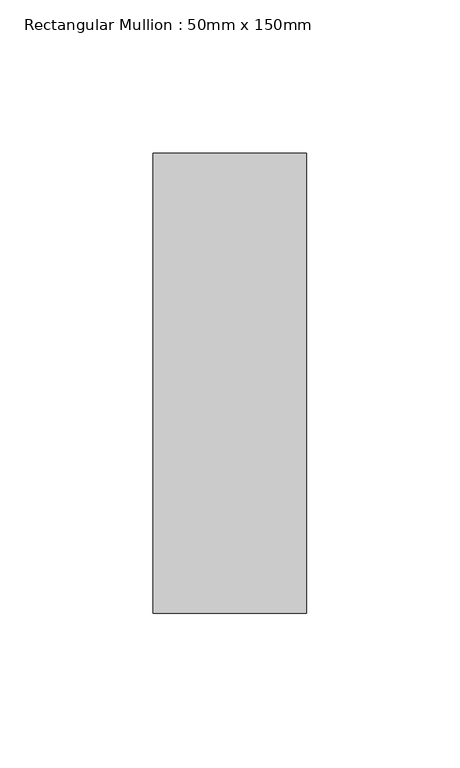
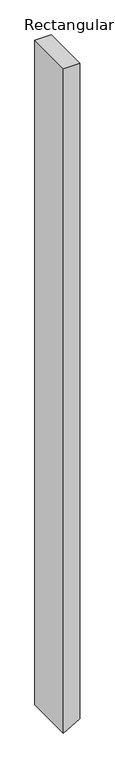
"""IFC4 building model written with IfcOpenShell, lengths in millimetres: member geometry, Rectangular Mullion : 50mm x 150mm."""

from ifc_helpers import new_model, si_unit, frame, origin, place, context, project, spatial, polyline, outline, extrude, source, transform, mapped, element, save


def rectangular_mullion_50mm_x_150mm_c4d7f9a4(model_context):
    return source(origin(), model_context, "Body", "SweptSolid", [
        extrude(outline(polyline([(0.0, 25.0), (0.0, -25.0), (-2134.1765467, -25.0), (-2105.3090332, 25.0), (0.0, 25.0)])), frame((0.0, -75.0, 0.0), z_axis=(0.0, 1.0, 0.0), x_axis=(0.0, 0.0, 1.0)), (0.0, 0.0, 1.0), 150.0),
    ])


if __name__ == "__main__":
    model = new_model("IFC4")
    model_context = context("Model", 3, world=origin())
    ifc_project = project(units=[si_unit("LENGTHUNIT", "METRE", prefix="MILLI")], contexts=[model_context])
    site = spatial("IfcSite", under=ifc_project)
    building = spatial("IfcBuilding", under=site)
    placement = place(None, origin())
    rectangular_mullion_50mm_x_150mm_shape = rectangular_mullion_50mm_x_150mm_c4d7f9a4(model_context)
    element("IfcMember", 1, ObjectType="Rectangular Mullion : 50mm x 150mm", at=placement, inside=building, context=model_context, shape_type="MappedRepresentation", body=[
        mapped(rectangular_mullion_50mm_x_150mm_shape, transform((0.0, 0.0, 0.0), x_axis=(1.0, 0.0, 0.0), y_axis=(0.0, 1.0, 0.0), z_axis=(0.0, 0.0, 1.0))),
    ])
    save(model, "model.ifc")

# Revit data of these elements
# Type "Rectangular Mullion : 50mm x 150mm"
#   built-in parameter 1007304 = 0.492126 (stored number, unit not read)
#   built-in parameter 1007301 = 0.082021 (stored number, unit not read)
#   built-in parameter 1007300 = 0.082021 (stored number, unit not read)
# Element 1 (IfcMember, "Rectangular Mullion : 50mm x 150mm")
#   Materials on its faces: "Aluminum"
# Materials
#   "Aluminum": class "Metal", colour RGB 247 247 247, transparency 0, Description = "Aluminum 6061", Cost = 0
